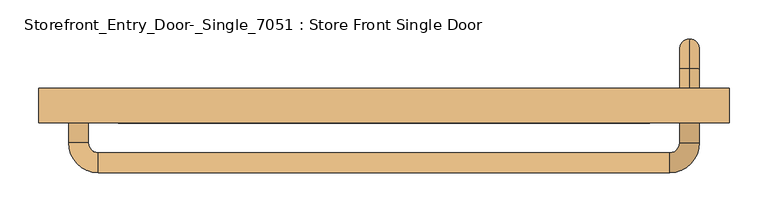
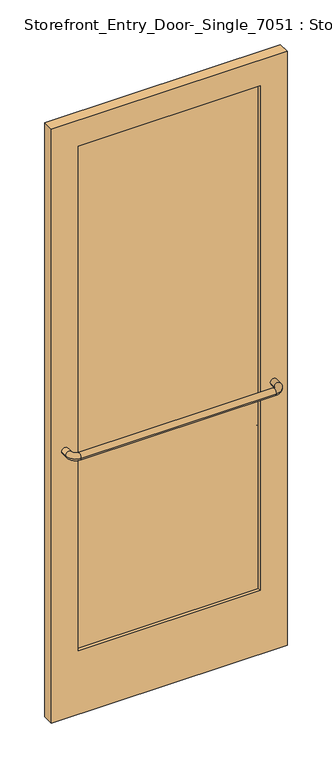
"""IFC4 building model written with IfcOpenShell, lengths in millimetres: door geometry, Storefront_Entry_Door-_Single_7051 : Store Front Single Door."""

import ifcopenshell
import ifcopenshell.guid

model = None  # the IFC model being written
_history = None  # IfcOwnerHistory: only IFC2X3 demands one
_inside = {}  # id of a spatial element -> (the spatial element, [elements in it])
_under = {}  # id of a project, library or spatial element -> (it, [spatial elements below it])
_declared = {}  # id of a project -> (the project, [libraries it declares])
_typed = {}  # id of a type object -> (the type object, [elements of that type])
_made_of = {}  # id of a material, layer set ... -> (it, [elements and type objects made of it])


def new_model(schema):
    """Start an empty IFC model of exactly this schema.

    Asked for "IFC4X3", IfcOpenShell would pick the latest addendum, in which some entities
    have other attributes; the version numbers below select the first issue.
    IFC2X3 requires an IfcOwnerHistory on every rooted entity: one is made here for all.
    """
    global model, _history
    if schema == "IFC4X3":
        model = ifcopenshell.file(schema_version=(4, 3, 0, 0))
    else:
        model = ifcopenshell.file(schema=schema)
    _inside.clear()
    _under.clear()
    _declared.clear()
    _typed.clear()
    _made_of.clear()
    _history = None
    if model.schema == "IFC2X3":
        org = make("IfcOrganization", Name="unknown")
        user = make(
            "IfcPersonAndOrganization",
            ThePerson=make("IfcPerson", FamilyName="unknown"),
            TheOrganization=org,
        )
        app = make(
            "IfcApplication",
            ApplicationDeveloper=org,
            Version="unknown",
            ApplicationFullName="unknown",
            ApplicationIdentifier="unknown",
        )
        _history = make(
            "IfcOwnerHistory",
            OwningUser=user,
            OwningApplication=app,
            ChangeAction="ADDED",
            CreationDate=0,
        )
    return model


def make(cls, **values):
    """One entity of the class cls with the attributes given. An attribute that is None is left unset."""
    return model.create_entity(
        cls, **{name: value for name, value in values.items() if value is not None}
    )


def rooted(cls, **values):
    """An entity with a GlobalId (a new one), such as an element, a storey or a relation."""
    return make(cls, GlobalId=ifcopenshell.guid.new(), OwnerHistory=_history, **values)


def si_unit(unit_type, name, prefix=None):
    """IfcSIUnit, for example si_unit("LENGTHUNIT", "METRE", prefix="MILLI")."""
    return make("IfcSIUnit", UnitType=unit_type, Prefix=prefix, Name=name)


def assignment(units):
    """IfcUnitAssignment: the units of a project."""
    return None if units is None else make("IfcUnitAssignment", Units=units)


def point(xyz):
    """IfcCartesianPoint."""
    return None if xyz is None else make("IfcCartesianPoint", Coordinates=xyz)


def direction(xyz):
    """IfcDirection."""
    return None if xyz is None else make("IfcDirection", DirectionRatios=xyz)


def frame(location, z_axis=None, x_axis=None):
    """IfcAxis2Placement3D, a coordinate frame: its origin and axes. An axis left out is left unset."""
    return make(
        "IfcAxis2Placement3D",
        Location=point(location),
        Axis=direction(z_axis),
        RefDirection=direction(x_axis),
    )


def origin():
    """The frame at (0, 0, 0) with its axes left unset."""
    return frame((0.0, 0.0, 0.0))


def place(relative_to, where):
    """IfcLocalPlacement: puts the frame where relative to a parent placement (None: the world)."""
    return make(
        "IfcLocalPlacement", PlacementRelTo=relative_to, RelativePlacement=where
    )


def context(
    kind, dimensions, precision=None, world=None, true_north=None, identifier=None
):
    """IfcGeometricRepresentationContext, for example the 3D "Model" context."""
    return make(
        "IfcGeometricRepresentationContext",
        ContextIdentifier=identifier,
        ContextType=kind,
        CoordinateSpaceDimension=dimensions,
        Precision=precision,
        WorldCoordinateSystem=world,
        TrueNorth=true_north,
    )


def project(units=None, contexts=None):
    """IfcProject with its units and contexts."""
    return rooted(
        "IfcProject",
        Name="project",
        RepresentationContexts=contexts,
        UnitsInContext=assignment(units),
    )


def spatial(cls, under=None, at=None, **own):
    """A site, building, storey or space (cls), placed at a placement, below another one or the project."""
    s = rooted(cls, ObjectPlacement=at, **own)
    if under is not None:
        _under.setdefault(under.id(), (under, []))[1].append(s)
    return s


def polyline(points):
    """IfcPolyline through the points."""
    return make("IfcPolyline", Points=[point(p) for p in points])


def circle_curve(where, radius):
    """IfcCircle in the frame where."""
    return make("IfcCircle", Position=where, Radius=radius)


def ellipse_curve(where, semi_axis1, semi_axis2):
    """IfcEllipse in the frame where."""
    return make(
        "IfcEllipse", Position=where, SemiAxis1=semi_axis1, SemiAxis2=semi_axis2
    )


def trimmed(basis, trim1, trim2, sense, master):
    """IfcTrimmedCurve: the piece of a basis curve between two trims."""
    return make(
        "IfcTrimmedCurve",
        BasisCurve=basis,
        Trim1=trim1,
        Trim2=trim2,
        SenseAgreement=sense,
        MasterRepresentation=master,
    )


def outline(outer, holes=None, kind="AREA"):
    """IfcArbitraryClosedProfileDef: a profile drawn as a closed curve; with holes, ...WithVoids."""
    if holes is None:
        return make("IfcArbitraryClosedProfileDef", ProfileType=kind, OuterCurve=outer)
    return make(
        "IfcArbitraryProfileDefWithVoids",
        ProfileType=kind,
        OuterCurve=outer,
        InnerCurves=holes,
    )


def extrude(swept, where, along, depth):
    """IfcExtrudedAreaSolid: the profile swept, set in the frame where, extruded along a direction by depth."""
    return make(
        "IfcExtrudedAreaSolid",
        SweptArea=swept,
        Position=where,
        ExtrudedDirection=direction(along),
        Depth=depth,
    )


def shape(context_of_items, identifier, shape_type, items):
    """IfcShapeRepresentation: the items that make up one representation, for example the "Body"."""
    return make(
        "IfcShapeRepresentation",
        ContextOfItems=context_of_items,
        RepresentationIdentifier=identifier,
        RepresentationType=shape_type,
        Items=items,
    )


def source(mapping_origin, context_of_items, identifier, shape_type, items):
    """IfcRepresentationMap: a shape defined once, which mapped items show again and again."""
    return make(
        "IfcRepresentationMap",
        MappingOrigin=mapping_origin,
        MappedRepresentation=shape(context_of_items, identifier, shape_type, items),
    )


def transform(
    local_origin,
    x_axis=None,
    y_axis=None,
    z_axis=None,
    scale=None,
    scale2=None,
    scale3=None,
    uniform=True,
):
    """IfcCartesianTransformationOperator3D, or its non-uniform kind. x_axis, y_axis, z_axis: its Axis1, 2, 3."""
    if uniform:
        return make(
            "IfcCartesianTransformationOperator3D",
            Axis1=direction(x_axis),
            Axis2=direction(y_axis),
            LocalOrigin=point(local_origin),
            Scale=scale,
            Axis3=direction(z_axis),
        )
    return make(
        "IfcCartesianTransformationOperator3DnonUniform",
        Axis1=direction(x_axis),
        Axis2=direction(y_axis),
        LocalOrigin=point(local_origin),
        Scale=scale,
        Axis3=direction(z_axis),
        Scale2=scale2,
        Scale3=scale3,
    )


def mapped(mapping_source, mapping_target):
    """IfcMappedItem: shows the shape of a source again, moved by a transform."""
    return make(
        "IfcMappedItem", MappingSource=mapping_source, MappingTarget=mapping_target
    )


def made_of(thing, what):
    """Note that an element or type object is made of a material, layer set ...; save() writes the relation."""
    if what is not None:
        _made_of.setdefault(what.id(), (what, []))[1].append(thing)
    return thing


def element(
    cls,
    number,
    at=None,
    inside=None,
    cuts=None,
    type_object=None,
    material=None,
    context=None,
    identifier="Body",
    shape_type=None,
    held_by="IfcProductDefinitionShape",
    body=None,
    shapes=None,
    **own,
):
    """One element of the class cls, such as IfcWall. Its Tag is "e" and its number.

    at: its placement. inside: the storey or other place that contains it. cuts: it is an
    opening in that element (IfcRelVoidsElement). A single representation is given by context,
    identifier, shape_type and body (its items); several are given by shapes. held_by: the class
    of the entity that holds the representations. save() writes the other relations.
    """
    e = rooted(cls, Tag="e%d" % number, ObjectPlacement=at, **own)
    if body is not None:
        shapes = [shape(context, identifier, shape_type, body)]
    if shapes is not None:
        e.Representation = make(held_by, Representations=shapes)
    if inside is not None:
        _inside.setdefault(inside.id(), (inside, []))[1].append(e)
    if cuts is not None:
        rooted(
            "IfcRelVoidsElement", RelatingBuildingElement=cuts, RelatedOpeningElement=e
        )
    if type_object is not None:
        _typed.setdefault(type_object.id(), (type_object, []))[1].append(e)
    return made_of(e, material)


def aggregate(whole, parts):
    """IfcRelAggregates: a whole, such as a stair, and the parts it consists of."""
    return rooted("IfcRelAggregates", RelatingObject=whole, RelatedObjects=parts)


def save(model, path):
    """Write the relations noted so far, then the file.

    IfcRelAggregates (storeys below a building ...), IfcRelContainedInSpatialStructure (elements
    in a storey), IfcRelDefinesByType, IfcRelAssociatesMaterial and IfcRelDeclares: one each for
    every whole, place, type object, material and project.
    """
    for whole, parts in _under.values():
        aggregate(whole, parts)
    for where, things in _inside.values():
        rooted(
            "IfcRelContainedInSpatialStructure",
            RelatedElements=things,
            RelatingStructure=where,
        )
    for kind, things in _typed.values():
        rooted("IfcRelDefinesByType", RelatedObjects=things, RelatingType=kind)
    for what, things in _made_of.values():
        rooted("IfcRelAssociatesMaterial", RelatedObjects=things, RelatingMaterial=what)
    for by, libraries in _declared.values():
        rooted("IfcRelDeclares", RelatingContext=by, RelatedDefinitions=libraries)
    model.write(path)


def plane_surface(at):
    """IfcPlane: the flat surface through the origin of the frame at, square to its z axis."""
    return make("IfcPlane", Position=at)


def cylinder_surface(at, radius):
    """IfcCylindricalSurface: all points at the distance radius from the z axis of the frame at."""
    return make("IfcCylindricalSurface", Position=at, Radius=radius)


def revolved_surface(curve, axis_point, axis_direction):
    """IfcSurfaceOfRevolution: the curve turned about the line through axis_point along axis_direction."""
    return make(
        "IfcSurfaceOfRevolution",
        SweptCurve=make("IfcArbitraryOpenProfileDef", ProfileType="CURVE", Curve=curve),
        AxisPosition=make("IfcAxis1Placement", Location=point(axis_point), Axis=direction(axis_direction)),
    )


def advanced_brep(points, edges, surfaces, faces):
    """IfcAdvancedBrep: a solid bounded by faces that lie on surfaces and meet in shared edges.

    An edge is (start, end): straight between two places in points (the first is 0);
    or (start, end, curve); or (start, end, curve, False) where it runs against its curve.
    A face is (place in surfaces, loops), or (place, loops, False) where it looks against
    its surface's normal. A loop lists edges by number (the first is 1), with a minus sign
    where the edge is run from its end to its start. The first loop is the outer one.
    """
    corners = [point(p) for p in points]
    vertices = [make("IfcVertexPoint", VertexGeometry=c) for c in corners]
    made = []
    for start, end, *more in edges:
        made.append(
            make(
                "IfcEdgeCurve",
                EdgeStart=vertices[start],
                EdgeEnd=vertices[end],
                EdgeGeometry=more[0] if more else make("IfcPolyline", Points=[corners[start], corners[end]]),
                SameSense=more[1] if len(more) > 1 else True,
            )
        )
    hull = []
    for where, loops, *sense in faces:
        bounds = []
        for j, loop in enumerate(loops):
            ring = [make("IfcOrientedEdge", EdgeElement=made[abs(k) - 1], Orientation=k > 0) for k in loop]
            bounds.append(
                make(
                    "IfcFaceOuterBound" if j == 0 else "IfcFaceBound",
                    Bound=make("IfcEdgeLoop", EdgeList=ring),
                    Orientation=True,
                )
            )
        hull.append(make("IfcAdvancedFace", Bounds=bounds, FaceSurface=surfaces[where], SameSense=sense[0] if sense else True))
    return make("IfcAdvancedBrep", Outer=make("IfcClosedShell", CfsFaces=hull))


def storefront_entry_door_single_7051_store_front_single_door_fded41a4(model_context):
    return source(origin(), model_context, "Body", "SolidModel", [
        advanced_brep(
        [(392.43, 50.8, 1054.1), (392.43, 50.8, 1079.5), (392.43, 76.2, 1054.1), (392.43, 76.2, 1079.5), (392.43, 114.3, 1041.4), (392.43, 88.9, 1041.4), (392.43, 88.9, 863.6), (392.43, 114.3, 863.6), (392.43, 76.2, 825.5), (392.43, 76.2, 850.9), (392.43, 50.8, 850.9), (392.43, 50.8, 825.5)],
        [
            (0, 1, circle_curve(frame((392.43, 50.8, 1066.8), z_axis=(0.0, -1.0, 0.0), x_axis=(0.0, 0.0, 1.0)), 12.7)),
            (1, 0, circle_curve(frame((392.43, 50.8, 1066.8), z_axis=(0.0, -1.0, 0.0), x_axis=(0.0, 0.0, 1.0)), 12.7)),
            (0, 2),
            (2, 3, circle_curve(frame((392.43, 76.2, 1066.8), z_axis=(0.0, -1.0, 0.0), x_axis=(0.0, 0.0, 1.0)), 12.7)),
            (3, 1),
            (3, 2, circle_curve(frame((392.43, 76.2, 1066.8), z_axis=(0.0, -1.0, 0.0), x_axis=(0.0, 0.0, 1.0)), 12.7)),
            (4, 3, circle_curve(frame((392.43, 76.2, 1041.4), z_axis=(1.0, 0.0, 0.0), x_axis=(0.0, 0.0, 1.0)), 38.1)),
            (2, 5, circle_curve(frame((392.43, 76.2, 1041.4), z_axis=(-1.0, 0.0, 0.0), x_axis=(0.0, 0.0, 1.0)), 12.7)),
            (5, 4, circle_curve(frame((392.43, 101.6, 1041.4), z_axis=(0.0, 0.0, 1.0), x_axis=(0.0, 1.0, 0.0)), 12.7)),
            (4, 5, circle_curve(frame((392.43, 101.6, 1041.4), z_axis=(0.0, 0.0, 1.0), x_axis=(0.0, 1.0, 0.0)), 12.7)),
            (5, 6),
            (6, 7, circle_curve(frame((392.43, 101.6, 863.6), z_axis=(0.0, 0.0, 1.0), x_axis=(0.0, 1.0, 0.0)), 12.7)),
            (7, 4),
            (7, 6, circle_curve(frame((392.43, 101.6, 863.6), z_axis=(0.0, 0.0, 1.0), x_axis=(0.0, 1.0, 0.0)), 12.7)),
            (8, 7, circle_curve(frame((392.43, 76.2, 863.6), z_axis=(1.0, 0.0, 0.0), x_axis=(0.0, 1.0, 0.0)), 38.1)),
            (6, 9, circle_curve(frame((392.43, 76.2, 863.6), z_axis=(-1.0, 0.0, 0.0), x_axis=(0.0, 1.0, 0.0)), 12.7)),
            (9, 8, circle_curve(frame((392.43, 76.2, 838.2), z_axis=(0.0, 1.0, 0.0), x_axis=(0.0, 0.0, -1.0)), 12.7)),
            (8, 9, circle_curve(frame((392.43, 76.2, 838.2), z_axis=(0.0, 1.0, 0.0), x_axis=(0.0, 0.0, -1.0)), 12.7)),
            (10, 11, circle_curve(frame((392.43, 50.8, 838.2), z_axis=(0.0, -1.0, 0.0), x_axis=(0.0, 0.0, -1.0)), 12.7)),
            (11, 10, circle_curve(frame((392.43, 50.8, 838.2), z_axis=(0.0, -1.0, 0.0), x_axis=(0.0, 0.0, -1.0)), 12.7)),
            (9, 10),
            (11, 8),
        ],
        [
            plane_surface(frame((392.43, 50.8, 1066.8), z_axis=(0.0, -1.0, 0.0), x_axis=(1.0, 0.0, 0.0))),
            cylinder_surface(frame((392.43, 50.8, 1066.8), z_axis=(0.0, -1.0, 0.0), x_axis=(0.0, 0.0, 1.0)), 12.7),
            revolved_surface(trimmed(ellipse_curve(frame((392.43, 76.2, 1066.8), z_axis=(0.0, -1.0, 0.0), x_axis=(0.0, 0.0, 1.0)), 12.7, 12.7), [point((392.43, 76.2, 1054.1))], [point((392.43, 76.2, 1079.5))], True, "CARTESIAN"), (392.43, 76.2, 1041.4), (-1.0, 0.0, 0.0)),
            revolved_surface(trimmed(ellipse_curve(frame((392.43, 76.2, 1066.8), z_axis=(0.0, -1.0, 0.0), x_axis=(0.0, 0.0, 1.0)), 12.7, 12.7), [point((392.43, 76.2, 1079.5))], [point((392.43, 76.2, 1054.1))], True, "CARTESIAN"), (392.43, 76.2, 1041.4), (-1.0, 0.0, 0.0)),
            cylinder_surface(frame((392.43, 101.6, 1041.4), z_axis=(0.0, 0.0, 1.0), x_axis=(0.0, 1.0, 0.0)), 12.7),
            revolved_surface(trimmed(ellipse_curve(frame((392.43, 101.6, 863.6), z_axis=(0.0, 0.0, 1.0), x_axis=(0.0, 1.0, 0.0)), 12.7, 12.7), [point((392.43, 88.9, 863.6))], [point((392.43, 114.3, 863.6))], True, "CARTESIAN"), (392.43, 76.2, 863.6), (-1.0, 0.0, 0.0)),
            revolved_surface(trimmed(ellipse_curve(frame((392.43, 101.6, 863.6), z_axis=(0.0, 0.0, 1.0), x_axis=(0.0, 1.0, 0.0)), 12.7, 12.7), [point((392.43, 114.3, 863.6))], [point((392.43, 88.9, 863.6))], True, "CARTESIAN"), (392.43, 76.2, 863.6), (-1.0, 0.0, 0.0)),
            plane_surface(frame((392.43, 50.8, 838.2), z_axis=(0.0, -1.0, 0.0), x_axis=(1.0, 0.0, 0.0))),
            cylinder_surface(frame((392.43, 76.2, 838.2), z_axis=(0.0, 1.0, 0.0), x_axis=(0.0, 0.0, -1.0)), 12.7),
        ],
        [
            (0, [[1, 2]]),
            (1, [[-1, 3, 4, 5]]),
            (1, [[-2, -5, 6, -3]]),
            (2, [[7, -4, 8, 9]]),
            (3, [[-8, -6, -7, 10]]),
            (4, [[-9, 11, 12, 13]]),
            (4, [[-10, -13, 14, -11]]),
            (5, [[15, -12, 16, 17]]),
            (6, [[-16, -14, -15, 18]]),
            (7, [[19, 20]]),
            (8, [[-17, 21, -20, 22]]),
            (8, [[-18, -22, -19, -21]]),
        ],
    ),
        advanced_brep(
        [(379.73, 6.35, 1066.8), (405.13, 6.35, 1066.8), (379.73, -19.05, 1066.8), (405.13, -19.05, 1066.8), (367.03, -57.15, 1066.8), (367.03, -31.75, 1066.8), (-367.03, -31.75, 1066.8), (-367.03, -57.15, 1066.8), (-405.13, -19.05, 1066.8), (-379.73, -19.05, 1066.8), (-379.73, 6.35, 1066.8), (-405.13, 6.35, 1066.8)],
        [
            (0, 1, circle_curve(frame((392.43, 6.35, 1066.8), z_axis=(0.0, 1.0, 0.0), x_axis=(1.0, 0.0, 0.0)), 12.7)),
            (1, 0, circle_curve(frame((392.43, 6.35, 1066.8), z_axis=(0.0, 1.0, 0.0), x_axis=(1.0, 0.0, 0.0)), 12.7)),
            (0, 2),
            (2, 3, circle_curve(frame((392.43, -19.05, 1066.8), z_axis=(0.0, 1.0, 0.0), x_axis=(1.0, 0.0, 0.0)), 12.7)),
            (3, 1),
            (3, 2, circle_curve(frame((392.43, -19.05, 1066.8), z_axis=(0.0, 1.0, 0.0), x_axis=(1.0, 0.0, 0.0)), 12.7)),
            (4, 3, circle_curve(frame((367.03, -19.05, 1066.8), z_axis=(0.0, 0.0, 1.0), x_axis=(1.0, 0.0, 0.0)), 38.1)),
            (2, 5, circle_curve(frame((367.03, -19.05, 1066.8), z_axis=(0.0, 0.0, -1.0), x_axis=(1.0, 0.0, 0.0)), 12.7)),
            (5, 4, circle_curve(frame((367.03, -44.45, 1066.8), z_axis=(1.0, 0.0, 0.0), x_axis=(0.0, -1.0, 0.0)), 12.7)),
            (4, 5, circle_curve(frame((367.03, -44.45, 1066.8), z_axis=(1.0, 0.0, 0.0), x_axis=(0.0, -1.0, 0.0)), 12.7)),
            (5, 6),
            (6, 7, circle_curve(frame((-367.03, -44.45, 1066.8), z_axis=(1.0, 0.0, 0.0), x_axis=(0.0, -1.0, 0.0)), 12.7)),
            (7, 4),
            (7, 6, circle_curve(frame((-367.03, -44.45, 1066.8), z_axis=(1.0, 0.0, 0.0), x_axis=(0.0, -1.0, 0.0)), 12.7)),
            (8, 7, circle_curve(frame((-367.03, -19.05, 1066.8), z_axis=(0.0, 0.0, 1.0), x_axis=(0.0, -1.0, 0.0)), 38.1)),
            (6, 9, circle_curve(frame((-367.03, -19.05, 1066.8), z_axis=(0.0, 0.0, -1.0), x_axis=(0.0, -1.0, 0.0)), 12.7)),
            (9, 8, circle_curve(frame((-392.43, -19.05, 1066.8), z_axis=(0.0, -1.0, 0.0), x_axis=(-1.0, 0.0, 0.0)), 12.7)),
            (8, 9, circle_curve(frame((-392.43, -19.05, 1066.8), z_axis=(0.0, -1.0, 0.0), x_axis=(-1.0, 0.0, 0.0)), 12.7)),
            (10, 11, circle_curve(frame((-392.43, 6.35, 1066.8), z_axis=(0.0, 1.0, 0.0), x_axis=(-1.0, 0.0, 0.0)), 12.7)),
            (11, 10, circle_curve(frame((-392.43, 6.35, 1066.8), z_axis=(0.0, 1.0, 0.0), x_axis=(-1.0, 0.0, 0.0)), 12.7)),
            (9, 10),
            (11, 8),
        ],
        [
            plane_surface(frame((392.43, 6.35, 1066.8), z_axis=(0.0, 1.0, 0.0), x_axis=(0.0, 0.0, 1.0))),
            cylinder_surface(frame((392.43, 6.35, 1066.8), z_axis=(0.0, 1.0, 0.0), x_axis=(1.0, 0.0, 0.0)), 12.7),
            revolved_surface(trimmed(ellipse_curve(frame((392.43, -19.05, 1066.8), z_axis=(0.0, 1.0, 0.0), x_axis=(1.0, 0.0, 0.0)), 12.7, 12.7), [point((379.73, -19.05, 1066.8))], [point((405.13, -19.05, 1066.8))], True, "CARTESIAN"), (367.03, -19.05, 1066.8), (0.0, 0.0, -1.0)),
            revolved_surface(trimmed(ellipse_curve(frame((392.43, -19.05, 1066.8), z_axis=(0.0, 1.0, 0.0), x_axis=(1.0, 0.0, 0.0)), 12.7, 12.7), [point((405.13, -19.05, 1066.8))], [point((379.73, -19.05, 1066.8))], True, "CARTESIAN"), (367.03, -19.05, 1066.8), (0.0, 0.0, -1.0)),
            cylinder_surface(frame((367.03, -44.45, 1066.8), z_axis=(1.0, 0.0, 0.0), x_axis=(0.0, -1.0, 0.0)), 12.7),
            revolved_surface(trimmed(ellipse_curve(frame((-367.03, -44.45, 1066.8), z_axis=(1.0, 0.0, 0.0), x_axis=(0.0, -1.0, 0.0)), 12.7, 12.7), [point((-367.03, -31.75, 1066.8))], [point((-367.03, -57.15, 1066.8))], True, "CARTESIAN"), (-367.03, -19.05, 1066.8), (0.0, 0.0, -1.0)),
            revolved_surface(trimmed(ellipse_curve(frame((-367.03, -44.45, 1066.8), z_axis=(1.0, 0.0, 0.0), x_axis=(0.0, -1.0, 0.0)), 12.7, 12.7), [point((-367.03, -57.15, 1066.8))], [point((-367.03, -31.75, 1066.8))], True, "CARTESIAN"), (-367.03, -19.05, 1066.8), (0.0, 0.0, -1.0)),
            plane_surface(frame((-392.43, 6.35, 1066.8), z_axis=(0.0, 1.0, 0.0), x_axis=(0.0, 0.0, 1.0))),
            cylinder_surface(frame((-392.43, -19.05, 1066.8), z_axis=(0.0, -1.0, 0.0), x_axis=(-1.0, 0.0, 0.0)), 12.7),
        ],
        [
            (0, [[1, 2]]),
            (1, [[-1, 3, 4, 5]]),
            (1, [[-2, -5, 6, -3]]),
            (2, [[7, -4, 8, 9]]),
            (3, [[-8, -6, -7, 10]]),
            (4, [[-9, 11, 12, 13]]),
            (4, [[-10, -13, 14, -11]]),
            (5, [[15, -12, 16, 17]]),
            (6, [[-16, -14, -15, 18]]),
            (7, [[19, 20]]),
            (8, [[-17, 21, -20, 22]]),
            (8, [[-18, -22, -19, -21]]),
        ],
    ),
        extrude(outline(polyline([(341.63, 19.05), (-341.63, 19.05), (-341.63, 38.1), (341.63, 38.1), (341.63, 19.05)])), frame((0.0, 0.0, 254.0), z_axis=(0.0, 0.0, 1.0), x_axis=(1.0, 0.0, 0.0)), (0.0, 0.0, 1.0), 2006.6),
        extrude(outline(polyline([(2362.2, 443.23), (2362.2, -443.23), (0.0, -443.23), (0.0, 443.23), (2362.2, 443.23)]), holes=[polyline([(2260.6, -341.63), (2260.6, 341.63), (254.0, 341.63), (254.0, -341.63), (2260.6, -341.63)])]), frame((0.0, 6.35, 0.0), z_axis=(0.0, 1.0, 0.0), x_axis=(0.0, 0.0, 1.0)), (0.0, 0.0, 1.0), 44.45),
    ])


if __name__ == "__main__":
    model = new_model("IFC4")
    model_context = context("Model", 3, world=origin())
    ifc_project = project(units=[si_unit("LENGTHUNIT", "METRE", prefix="MILLI")], contexts=[model_context])
    site = spatial("IfcSite", under=ifc_project)
    building = spatial("IfcBuilding", under=site)
    placement = place(None, origin())
    storefront_entry_door_single_7051_store_front_single_door_shape = storefront_entry_door_single_7051_store_front_single_door_fded41a4(model_context)
    element("IfcDoor", 1, ObjectType="Storefront_Entry_Door-_Single_7051 : Store Front Single Door", at=placement, inside=building, context=model_context, shape_type="MappedRepresentation", body=[
        mapped(storefront_entry_door_single_7051_store_front_single_door_shape, transform((0.0, 0.0, 0.0), x_axis=(1.0, 0.0, 0.0), y_axis=(0.0, 1.0, 0.0), z_axis=(0.0, 0.0, 1.0))),
    ])
    save(model, "model.ifc")

# Revit data of these elements
# Type "Storefront_Entry_Door-_Single_7051 : Store Front Single Door"
#   Type Comments = "TEMPERED GLAZING"
#   Type Mark = "19"
#   Assembly Code = "B2030110"
#   Analytic Construction = "<None>"
#   Top Rail = 0' - 4"
#   Side Rail = 0' - 4"
#   Reporting Width [instance default] = 4' - 2"
#   Rail Height AFF = 3' - 6"
#   Offset = 0' - 2"
#   Door Width [instance default] = 4' - 2"
#   Bottom Rail Width = 0' - 10"
#   Material = Metal - Aluminum
#   Glazing Material = Glass
#   Function = (empty or 0)
# Element 1 (IfcDoor, "Storefront_Entry_Door-_Single_7051 : Store Front Single Door")
#   Reporting Width = 2' - 10.9"
#   Door Width = 2' - 10.9"
#   Materials on its faces: "Metal - Aluminum", "Glass"
# Materials
#   "Metal - Aluminum": class "Metal", colour RGB 247 247 247, transparency 0
#   "Glass": class "Glass", colour RGB 218 227 224, transparency 0.85, Description = "Soda Lime Glass", Cost = 0
